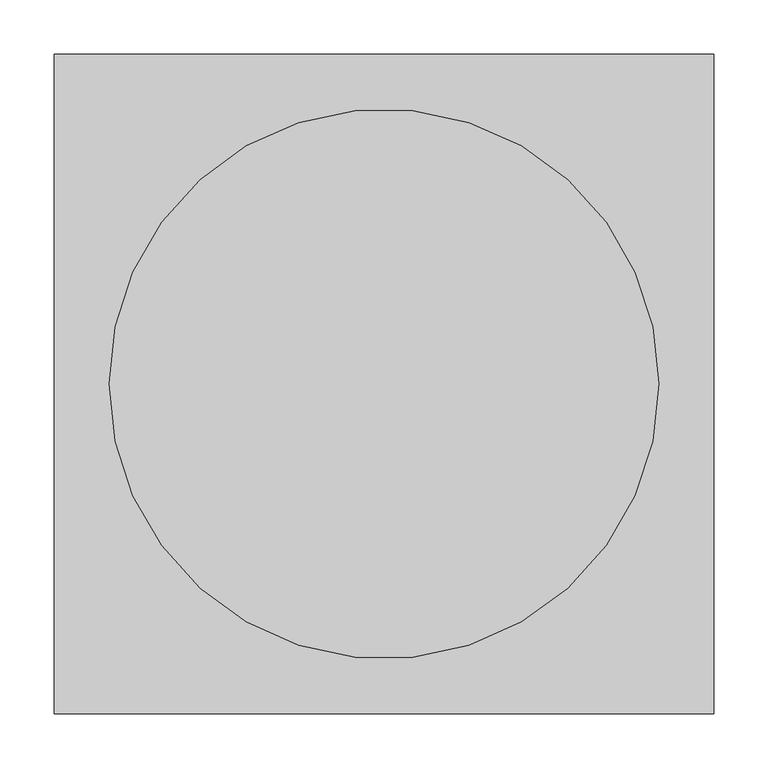
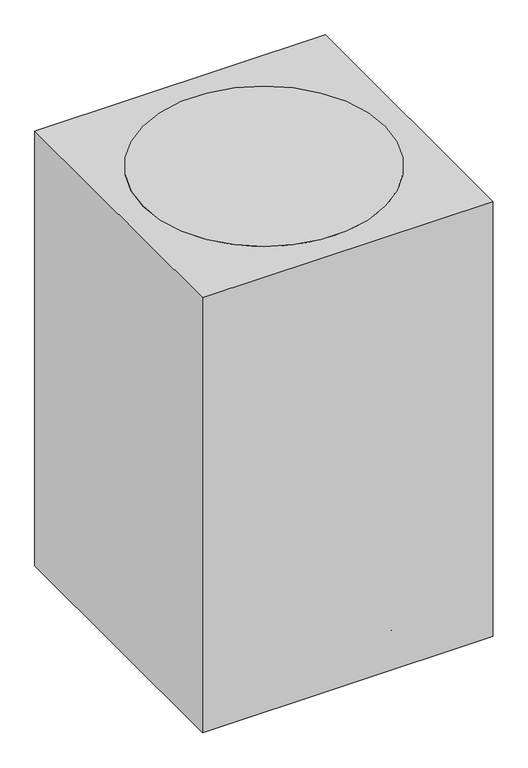
"""IFC4 building model written with IfcOpenShell, lengths in millimetres: proxy geometry, F0340 - Stool, Self Adjusting : F0340 - Stool, Self Adjusting."""

from ifc_helpers import new_model, si_unit, point, frame, frame_2d, origin, origin_with_axes, origin_2d, place, context, project, spatial, polyline, circle_curve, trimmed, segment, composite_curve, outline, extrude, source, transform, mapped, element, save


def specialty_equipment_b6c2791e(model_context):
    return source(origin(), model_context, "Body", "SweptSolid", [
        extrude(outline(composite_curve([segment(trimmed(circle_curve(frame_2d((0.0, -25.7612183)), 25.7612183), [point((0.0, -51.5224365))], [point((0.0, 0.0))], False, "CARTESIAN"), True, "CONTINUOUS"), segment(trimmed(circle_curve(frame_2d((0.0, -25.7612183)), 25.7612183), [point((0.0, 0.0))], [point((0.0, -51.5224365))], False, "CARTESIAN"), True, "CONTINUOUS")], self_intersect=False)), frame((203.8559823, 49.544861, 25.7612183), z_axis=(-0.3090169943748919, 0.9510565162951716, 0.0), x_axis=(0.0, 0.0, -1.0)), (0.0, 0.0, 1.0), 31.75),
        extrude(outline(composite_curve([segment(polyline([(-57.1058784, 0.0), (-0.678315, 0.0)]), True, "CONTINUOUS"), segment(trimmed(circle_curve(frame_2d((-28.8920968, 0.0)), 28.2137817), [point((-0.678315, 0.0))], [point((-57.1058784, 0.0))], False, "CARTESIAN"), True, "CONTINUOUS")], self_intersect=False)), frame((256.8155026, 63.4140597, 25.7612183), z_axis=(-0.30901699437489183, 0.9510565162951716, 0.0), x_axis=(0.9510565162951716, 0.30901699437489183, 0.0)), (0.0, 0.0, 1.0), 38.1),
        extrude(outline(composite_curve([segment(trimmed(circle_curve(frame_2d((223.4509477, 72.6028121)), 3.5091751), [point((222.3665529, 75.940236))], [point((224.5353424, 69.2653883))], False, "CARTESIAN"), True, "CONTINUOUS"), segment(trimmed(circle_curve(frame_2d((223.4509477, 72.6028121)), 3.5091751), [point((224.5353424, 69.2653883))], [point((222.3665529, 75.940236))], False, "CARTESIAN"), True, "CONTINUOUS")], self_intersect=False)), frame((0.0, 0.0, 53.975), z_axis=(0.0, 0.0, 1.0), x_axis=(1.0, 0.0, 0.0)), (0.0, 0.0, 1.0), 13.49375),
        extrude(outline(polyline([(230.0293313, 68.0638809), (25.3978935, 1.5750963), (21.4736172, 13.6527769), (226.105055, 80.1415615), (230.0293313, 68.0638809)])), frame((0.0, 0.0, 67.46875), z_axis=(0.0, 0.0, 1.0), x_axis=(1.0, 0.0, 0.0)), (0.0, 0.0, 1.0), 50.8),
        extrude(outline(composite_curve([segment(trimmed(circle_curve(frame_2d((0.0, -25.7612182)), 25.7612183), [point((0.0, -51.5224365))], [point((0.0, 0.0))], False, "CARTESIAN"), True, "CONTINUOUS"), segment(trimmed(circle_curve(frame_2d((0.0, -25.7612182)), 25.7612183), [point((0.0, 0.0))], [point((0.0, -51.5224365))], False, "CARTESIAN"), True, "CONTINUOUS")], self_intersect=False)), frame((110.1149259, -178.5683563, 25.7612183), z_axis=(0.8090169943749846, 0.5877852522924221, 0.0), x_axis=(0.0, 0.0, -1.0)), (0.0, 0.0, 1.0), 31.75),
        extrude(outline(composite_curve([segment(polyline([(-57.1058785, 0.0), (-0.6783149, 0.0)]), True, "CONTINUOUS"), segment(trimmed(circle_curve(frame_2d((-28.8920966, 0.0)), 28.2137817), [point((-0.6783149, 0.0))], [point((-57.1058785, 0.0))], False, "CARTESIAN"), True, "CONTINUOUS")], self_intersect=False)), frame((139.6707094, -224.6500351, 25.7612183), z_axis=(0.8090169943749845, 0.5877852522924222, 0.0), x_axis=(0.5877852522924222, -0.8090169943749845, 0.0)), (0.0, 0.0, 1.0), 38.1),
        extrude(outline(composite_curve([segment(trimmed(circle_curve(frame_2d((138.0995178, -190.0789771)), 3.5091751), [point((140.9385001, -188.0163357))], [point((135.2605355, -192.1416185))], False, "CARTESIAN"), True, "CONTINUOUS"), segment(trimmed(circle_curve(frame_2d((138.0995178, -190.0789771)), 3.5091751), [point((135.2605355, -192.1416185))], [point((140.9385001, -188.0163357))], False, "CARTESIAN"), True, "CONTINUOUS")], self_intersect=False)), frame((0.0, 0.0, 53.975), z_axis=(0.0, 0.0, 1.0), x_axis=(1.0, 0.0, 0.0)), (0.0, 0.0, 1.0), 13.49375),
        extrude(outline(polyline([(135.81557, -197.7379985), (9.3463863, -23.6681006), (19.620275, -16.2036835), (146.0894588, -190.2735815), (135.81557, -197.7379985)])), frame((0.0, 0.0, 67.46875), z_axis=(0.0, 0.0, 1.0), x_axis=(1.0, 0.0, 0.0)), (0.0, 0.0, 1.0), 50.8),
        extrude(outline(composite_curve([segment(trimmed(circle_curve(frame_2d((0.0, -25.7612182)), 25.7612183), [point((0.0, -51.5224365))], [point((0.0, 0.0))], False, "CARTESIAN"), True, "CONTINUOUS"), segment(trimmed(circle_curve(frame_2d((0.0, -25.7612182)), 25.7612183), [point((0.0, 0.0))], [point((0.0, -51.5224365))], False, "CARTESIAN"), True, "CONTINUOUS")], self_intersect=False)), frame((-110.1149259, -178.5683563, 25.7612183), z_axis=(-0.8090169943749151, 0.5877852522925178, 0.0), x_axis=(0.0, 0.0, 1.0)), (0.0, 0.0, 1.0), 31.75),
        extrude(outline(composite_curve([segment(trimmed(circle_curve(frame_2d((28.8920966, 0.0)), 28.2137817), [point((57.1058785, 0.0))], [point((0.6783149, 0.0))], False, "CARTESIAN"), True, "CONTINUOUS"), segment(polyline([(0.6783149, 0.0), (57.1058785, 0.0)]), True, "CONTINUOUS")], self_intersect=False)), frame((-139.6707094, -224.6500351, 25.7612183), z_axis=(-0.809016994374915, 0.5877852522925177, 0.0), x_axis=(0.5877852522925177, 0.809016994374915, 0.0)), (0.0, 0.0, 1.0), 38.1),
        extrude(outline(composite_curve([segment(trimmed(circle_curve(frame_2d((-138.1007518, -190.0780805)), 3.5091751), [point((-135.2617695, -192.1407219))], [point((-140.9397341, -188.0154391))], False, "CARTESIAN"), True, "CONTINUOUS"), segment(trimmed(circle_curve(frame_2d((-138.1007518, -190.0780805)), 3.5091751), [point((-140.9397341, -188.0154391))], [point((-135.2617695, -192.1407219))], False, "CARTESIAN"), True, "CONTINUOUS")], self_intersect=False)), frame((0.0, 0.0, 53.975), z_axis=(0.0, 0.0, 1.0), x_axis=(1.0, 0.0, 0.0)), (0.0, 0.0, 1.0), 13.49375),
        extrude(outline(polyline([(-146.0906928, -190.2726849), (-19.6215091, -16.2027869), (-9.3476203, -23.667204), (-135.8168041, -197.737102), (-146.0906928, -190.2726849)])), frame((0.0, 0.0, 67.46875), z_axis=(0.0, 0.0, 1.0), x_axis=(1.0, 0.0, 0.0)), (0.0, 0.0, 1.0), 50.8),
        extrude(outline(composite_curve([segment(trimmed(circle_curve(frame_2d((0.0, -25.7612183)), 25.7612183), [point((0.0, -51.5224365))], [point((0.0, 0.0))], False, "CARTESIAN"), True, "CONTINUOUS"), segment(trimmed(circle_curve(frame_2d((0.0, -25.7612183)), 25.7612183), [point((0.0, 0.0))], [point((0.0, -51.5224365))], False, "CARTESIAN"), True, "CONTINUOUS")], self_intersect=False)), frame((-203.8559823, 49.544861, 25.7612183), z_axis=(0.3090169943749793, 0.9510565162951433, 0.0), x_axis=(0.0, 0.0, 1.0)), (0.0, 0.0, 1.0), 31.75),
        extrude(outline(composite_curve([segment(trimmed(circle_curve(frame_2d((28.8920968, 0.0)), 28.2137817), [point((57.1058784, 0.0))], [point((0.678315, 0.0))], False, "CARTESIAN"), True, "CONTINUOUS"), segment(polyline([(0.678315, 0.0), (57.1058784, 0.0)]), True, "CONTINUOUS")], self_intersect=False)), frame((-256.8155026, 63.4140597, 25.7612183), z_axis=(0.3090169943749793, 0.9510565162951433, 0.0), x_axis=(0.9510565162951433, -0.3090169943749793, 0.0)), (0.0, 0.0, 1.0), 38.1),
        extrude(outline(composite_curve([segment(trimmed(circle_curve(frame_2d((-223.4504763, 72.6042628)), 3.5091751), [point((-224.5348711, 69.266839))], [point((-222.3660816, 75.9416867))], False, "CARTESIAN"), True, "CONTINUOUS"), segment(trimmed(circle_curve(frame_2d((-223.4504763, 72.6042628)), 3.5091751), [point((-222.3660816, 75.9416867))], [point((-224.5348711, 69.266839))], False, "CARTESIAN"), True, "CONTINUOUS")], self_intersect=False)), frame((0.0, 0.0, 53.975), z_axis=(0.0, 0.0, 1.0), x_axis=(1.0, 0.0, 0.0)), (0.0, 0.0, 1.0), 13.49375),
        extrude(outline(polyline([(-226.1045836, 80.1430121), (-21.4731458, 13.6542275), (-25.3974221, 1.576547), (-230.0288599, 68.0653316), (-226.1045836, 80.1430121)])), frame((0.0, 0.0, 67.46875), z_axis=(0.0, 0.0, 1.0), x_axis=(1.0, 0.0, 0.0)), (0.0, 0.0, 1.0), 50.8),
        extrude(outline(composite_curve([segment(trimmed(circle_curve(frame_2d((234.9499827, 25.7612183)), 25.7612183), [point((260.7112009, 25.7612183))], [point((209.1887644, 25.7612183))], False, "CARTESIAN"), True, "CONTINUOUS"), segment(trimmed(circle_curve(frame_2d((234.9499827, 25.7612183)), 25.7612183), [point((209.1887644, 25.7612183))], [point((260.7112009, 25.7612183))], False, "CARTESIAN"), True, "CONTINUOUS")], self_intersect=False)), frame((-15.875, 0.0, 0.0), z_axis=(1.0, 0.0, 0.0), x_axis=(0.0, 1.0, 0.0)), (0.0, 0.0, 1.0), 31.75),
        extrude(outline(composite_curve([segment(trimmed(circle_curve(frame_2d((234.9499827, 25.7612183)), 28.2137817), [point((206.7362009, 25.7612183))], [point((263.1637644, 25.7612183))], False, "CARTESIAN"), True, "CONTINUOUS"), segment(polyline([(263.1637644, 25.7612183), (206.7362009, 25.7612183)]), True, "CONTINUOUS")], self_intersect=False)), frame((-19.05, 0.0, 0.0), z_axis=(1.0, 0.0, 0.0), x_axis=(0.0, 1.0, 0.0)), (0.0, 0.0, 1.0), 38.1),
        extrude(outline(composite_curve([segment(trimmed(circle_curve(frame_2d((0.0007627, 234.9499827)), 3.5091751), [point((-3.5084124, 234.9499827))], [point((3.5099378, 234.9499827))], False, "CARTESIAN"), True, "CONTINUOUS"), segment(trimmed(circle_curve(frame_2d((0.0007627, 234.9499827)), 3.5091751), [point((3.5099378, 234.9499827))], [point((-3.5084124, 234.9499827))], False, "CARTESIAN"), True, "CONTINUOUS")], self_intersect=False)), frame((0.0, 0.0, 53.975), z_axis=(0.0, 0.0, 1.0), x_axis=(1.0, 0.0, 0.0)), (0.0, 0.0, 1.0), 13.49375),
        extrude(outline(polyline([(6.3503751, 239.8037904), (6.3503751, 24.6415636), (-6.3488498, 24.6415636), (-6.3488498, 239.8037904), (6.3503751, 239.8037904)])), frame((0.0, 0.0, 67.46875), z_axis=(0.0, 0.0, 1.0), x_axis=(1.0, 0.0, 0.0)), (0.0, 0.0, 1.0), 50.8),
        extrude(outline(composite_curve([segment(trimmed(circle_curve(origin_2d(), 25.4466483), [point((-25.4466483, 0.0))], [point((25.4466483, 0.0))], False, "CARTESIAN"), True, "CONTINUOUS"), segment(trimmed(circle_curve(origin_2d(), 25.4466483), [point((25.4466483, 0.0))], [point((-25.4466483, 0.0))], False, "CARTESIAN"), True, "CONTINUOUS")], self_intersect=False)), frame((0.0, 0.0, 67.46875), z_axis=(0.0, 0.0, 1.0), x_axis=(1.0, 0.0, 0.0)), (0.0, 0.0, 1.0), 846.93125),
        extrude(outline(composite_curve([segment(trimmed(circle_curve(origin_2d(), 254.0), [point((-254.0, 0.0))], [point((254.0, 0.0))], False, "CARTESIAN"), True, "CONTINUOUS"), segment(trimmed(circle_curve(origin_2d(), 254.0), [point((254.0, 0.0))], [point((-254.0, 0.0))], False, "CARTESIAN"), True, "CONTINUOUS")], self_intersect=False)), frame((0.0, 0.0, 914.4), z_axis=(0.0, 0.0, 1.0), x_axis=(1.0, 0.0, 0.0)), (0.0, 0.0, 1.0), 50.8),
        extrude(outline(polyline([(304.8, 304.8), (304.8, -304.8), (-304.8, -304.8), (-304.8, 304.8), (304.8, 304.8)])), origin_with_axes(), (0.0, 0.0, 1.0), 965.2),
    ])


if __name__ == "__main__":
    model = new_model("IFC4")
    model_context = context("Model", 3, world=origin())
    ifc_project = project(units=[si_unit("LENGTHUNIT", "METRE", prefix="MILLI")], contexts=[model_context])
    site = spatial("IfcSite", under=ifc_project)
    building = spatial("IfcBuilding", under=site)
    placement = place(None, origin())
    specialty_equipment_shape = specialty_equipment_b6c2791e(model_context)
    element("IfcBuildingElementProxy", 1, Name="F0340 - Stool, Self Adjusting : F0340 - Stool, Self Adjusting", ObjectType="F0340 - Stool, Self Adjusting : F0340 - Stool, Self Adjusting", at=placement, inside=building, context=model_context, shape_type="MappedRepresentation", body=[
        mapped(specialty_equipment_shape, transform((0.0, 0.0, 0.0), x_axis=(1.0, 0.0, 0.0), y_axis=(0.0, 1.0, 0.0), z_axis=(0.0, 0.0, 1.0))),
    ])
    save(model, "model.ifc")

# Revit data of these elements
# Type "F0340 - Stool, Self Adjusting : F0340 - Stool, Self Adjusting"
#   Watts2 = "0"
#   Watts1 = "0"
#   Unit_Issue = "EA"
#   UTIL_6_Misc = "-"
#   UTIL_5_NonMedGas = "-"
#   UTIL_4_MiscGas = "-"
#   UTIL_3_MedGas = "-"
#   UTIL_2_Elec = "-"
#   UTIL_1_WaterDrain = "-"
#   Nomenclature = "Stool, Self Adjusting"
#   NSN = "6530"
#   Location [instance default] = ""
#   JSN = "F0340"
#   Fund_Source_VA = "-"
#   Fund_Source_Navy = "-"
#   Fund_Source_Army = "-"
#   Fund_Source_AF = "-"
#   ELEC_Volts2 = "0"
#   ELEC_Volts1 = "0"
#   ELEC_Phase2 = "0"
#   ELEC_Phase1 = "0"
#   ELEC_HertzSwitch = "0"
#   ELEC_HertzDependent = "0"
#   ELEC_Hertz = "0"
#   ELEC_Amps2 = "0"
#   ELEC_Amps1 = "0"
#   DetailDescription = "Self adjusting stool. Consists of a foam padded upholstered seat with attached foot rest for added comfort. Mounted on swivel casters.  Designed for doctor''s use during examinations."
#   CAT_VA = "C"
#   CAT_Navy = "C"
#   CAT_IHS = "-"
#   CAT_Army = "C"
#   CAT_AF = "C"
#   BTUperhour = "0"
#   Weight_IP = 39
#   DIM_Width_IP = 2' - 0"
#   DIM_Height_IP = 3' - 2"
#   DIM_Depth_IP = 2' - 0"
#   Assembly Code = ""
# Element 1 (IfcBuildingElementProxy, "F0340 - Stool, Self Adjusting : F0340 - Stool, Self Adjusting")
#   Location = "OPCR2"
#   Materials on its faces: "Stool metal", "Stool caster", "EquipSpace", "Stool cushion"
# Materials
#   "Stool metal": class "Unassigned", colour RGB 201 201 201, transparency 0, Comments = "Rendering appearance not upgraded "
#   "Stool caster": class "Unassigned", colour RGB 0 0 0, transparency 0, Comments = "Rendering appearance not upgraded "
#   "EquipSpace": class "Unassigned", colour RGB 221 217 195, transparency 0.5
#   "Stool cushion": class "Unassigned", colour RGB 226 128 109, transparency 0, Comments = "Rendering appearance not upgraded "
